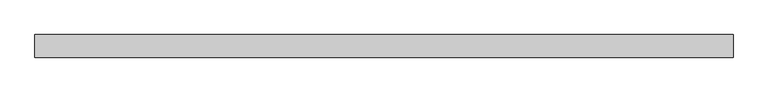
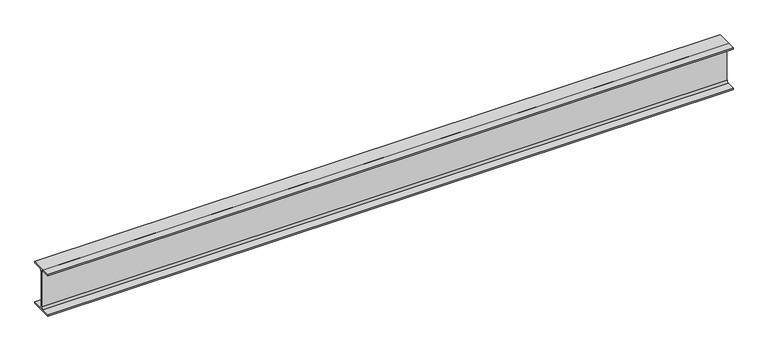
"""IFC4 building model written with IfcOpenShell, lengths in millimetres: beam geometry, 0912_Steel Framing_H-KSD3502 : H_SB_ASB_H-250x125x6x9."""

from ifc_helpers import new_model, si_unit, point, frame, frame_2d, origin, place, context, project, spatial, polyline, circle_curve, trimmed, segment, composite_curve, outline, extrude, source, transform, mapped, element, save


def beam_9772241e(model_context):
    return source(origin(), model_context, "Body", "SweptSolid", [
        extrude(outline(composite_curve([segment(polyline([(62.5, -116.0), (62.5, -125.0), (-62.5, -125.0), (-62.5, -116.0), (-15.0, -116.0)]), True, "CONTINUOUS"), segment(trimmed(circle_curve(frame_2d((-15.0, -104.0)), 12.0), [point((-15.0, -116.0))], [point((-3.0, -104.0))], True, "CARTESIAN"), True, "CONTINUOUS"), segment(polyline([(-3.0, -104.0), (-3.0, 104.0)]), True, "CONTINUOUS"), segment(trimmed(circle_curve(frame_2d((-15.0, 104.0)), 12.0), [point((-3.0, 104.0))], [point((-15.0, 116.0))], True, "CARTESIAN"), True, "CONTINUOUS"), segment(polyline([(-15.0, 116.0), (-62.5, 116.0), (-62.5, 125.0), (62.5, 125.0), (62.5, 116.0), (15.0, 116.0)]), True, "CONTINUOUS"), segment(trimmed(circle_curve(frame_2d((15.0, 104.0)), 12.0), [point((15.0, 116.0))], [point((3.0, 104.0))], True, "CARTESIAN"), True, "CONTINUOUS"), segment(polyline([(3.0, 104.0), (3.0, -104.0)]), True, "CONTINUOUS"), segment(trimmed(circle_curve(frame_2d((15.0, -104.0)), 12.0), [point((3.0, -104.0))], [point((15.0, -116.0))], True, "CARTESIAN"), True, "CONTINUOUS"), segment(polyline([(15.0, -116.0), (62.5, -116.0)]), True, "CONTINUOUS")], self_intersect=False)), frame((-1830.0827532, 0.0, 0.0), z_axis=(1.0, 0.0, 0.0), x_axis=(0.0, 1.0, 0.0)), (0.0, 0.0, 1.0), 3859.8827532),
    ])


if __name__ == "__main__":
    model = new_model("IFC4")
    model_context = context("Model", 3, world=origin())
    ifc_project = project(units=[si_unit("LENGTHUNIT", "METRE", prefix="MILLI")], contexts=[model_context])
    site = spatial("IfcSite", under=ifc_project)
    building = spatial("IfcBuilding", under=site)
    placement = place(None, origin())
    beam_shape = beam_9772241e(model_context)
    element("IfcBeam", 1, ObjectType="0912_Steel Framing_H-KSD3502 : H_SB_ASB_H-250x125x6x9", at=placement, inside=building, context=model_context, shape_type="MappedRepresentation", body=[
        mapped(beam_shape, transform((0.0, 0.0, 0.0), x_axis=(1.0, 0.0, 0.0), y_axis=(0.0, 1.0, 0.0), z_axis=(0.0, 0.0, 1.0))),
    ])
    save(model, "model.ifc")

# Revit data of these elements
# Type "0912_Steel Framing_H-KSD3502 : H_SB_ASB_H-250x125x6x9"
#   H_WM Code_1 = "S01AA003-00001 | Main Steel Structure Fabrication Work | Shelter/Building | Light Steel - Standard (30KG/M>Weight) | Material: (   )"
#   H_WM Code_2 = "S03AA029-00001 | Main Steel Structure Erection Work | Shelter/Building | Light Steel (30KG/M>Weight) | Material: (   )"
#   H_WM Code_3 = "S01AA010-00001 | Main Steel Structure Fabrication Work | Shelter/Building | Steel Painting/Coating | for Non-Fireproofed Steel Surface, Surface Preparation, Primer, Second & Final Coat | Material: (   )"
#   H_Q'ty Cal Type Tag = "SB-Q2"
#   Width = 12.5 cm
#   Web Thickness = 0.6 cm
#   Web Fillet = 1.2 cm
#   Warping Constant = 42539.8 cm⁶
#   W = 0
#   Torsional Moment of Inertia = 7.8102 cm⁴
#   Section Area = 37.66 cm²
#   Plastic Modulus weak axis = 73.1 cm³
#   Plastic Modulus strong axis = 366.0 cm³
#   Perimeter = 0.97 m²/m
#   Nominal Weight = 29.60 kgf/m
#   Moment of Inertia weak axis = 294.00 cm⁴
#   Moment of Inertia strong axis = 4050.00 cm⁴
#   Height = 25.0 cm
#   Flange Thickness = 0.9 cm
#   Elastic Modulus weak axis = 47.0 cm³
#   Elastic Modulus strong axis = 324.0 cm³
#   Centroid Vertical = 12.5 cm
#   Centroid Horizontal = 6.25 cm
#   Ix = 40500000
#   Length [instance default] = 1.5240 m
#   Zx = 366000
#   b = 0.1250 m
#   h = 0.2500 m
#   r = 0.0120 m
#   s = 0.0060 m
#   t = 0.0090 m
#   A = 0.003766 m²
#   Structural Material [instance default] = Steel, 45-345
#   Assembly Code = ""
# Element 1 (IfcBeam, "0912_Steel Framing_H-KSD3502 : H_SB_ASB_H-250x125x6x9")
#   Structural Material = none
# Materials
#   "Steel, 45-345": class "Metal", colour RGB 189 187 185, transparency 0, Description = "Steel 345 MPa", Cost = 0
